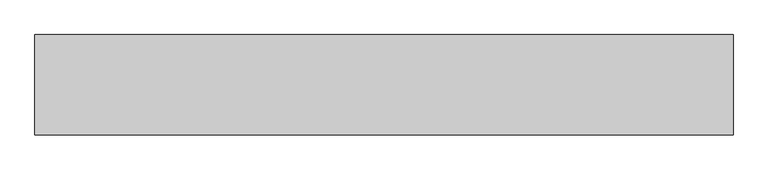
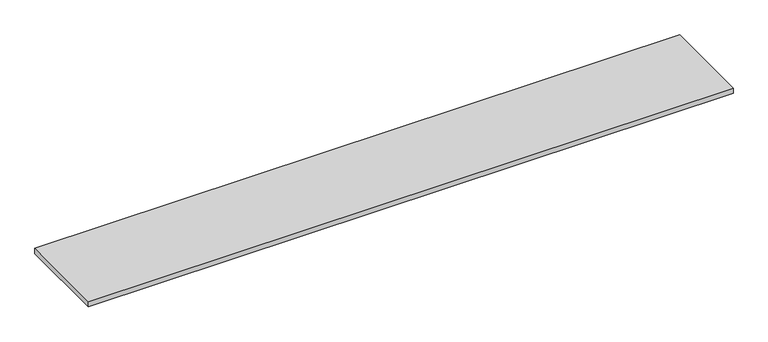
"""IFC4 building model written with IfcOpenShell, lengths in millimetres: furniture geometry, OD_CW_Countertop : OD_CW_Countertop."""

from ifc_helpers import new_model, si_unit, frame, origin, place, context, project, spatial, polyline, outline, extrude, source, transform, mapped, element, save


def furniture_1b7fe929(model_context):
    return source(origin(), model_context, "Body", "SweptSolid", [
        extrude(outline(polyline([(18.7377049, -609.6), (18.7377049, 25.4), (4438.3377049, 25.4), (4438.3377049, -609.6), (18.7377049, -609.6)])), frame((0.0, 0.0, 965.2), z_axis=(0.0, 0.0, 1.0), x_axis=(1.0, 0.0, 0.0)), (0.0, 0.0, 1.0), 38.1),
    ])


if __name__ == "__main__":
    model = new_model("IFC4")
    model_context = context("Model", 3, world=origin())
    ifc_project = project(units=[si_unit("LENGTHUNIT", "METRE", prefix="MILLI")], contexts=[model_context])
    site = spatial("IfcSite", under=ifc_project)
    building = spatial("IfcBuilding", under=site)
    placement = place(None, origin())
    furniture_shape = furniture_1b7fe929(model_context)
    element("IfcFurniture", 1, ObjectType="OD_CW_Countertop : OD_CW_Countertop", at=placement, inside=building, context=model_context, shape_type="MappedRepresentation", body=[
        mapped(furniture_shape, transform((0.0, 0.0, 0.0), x_axis=(1.0, 0.0, 0.0), y_axis=(0.0, 1.0, 0.0), z_axis=(0.0, 0.0, 1.0))),
    ])
    save(model, "model.ifc")

# Revit data of these elements
# Type "OD_CW_Countertop : OD_CW_Countertop"
#   OD_CW_Width [instance default] = 2' - 9"
#   OD_CW_Off Floor [instance default] = 3' - 2"
#   OD_CW_Length [instance default] = 6' - 9"
#   OD_CW_Height [instance default] = 7' - 0"
#   Depth = 2' - 0"
#   Height = 3' - 0"
#   Width = 4' - 0"
#   OD_CW_Material_Countertop [instance default] = none
# Element 1 (IfcFurniture, "OD_CW_Countertop : OD_CW_Countertop")
#   OD_CW_Width = 2' - 1"
#   OD_CW_Length = 14' - 6"
#   OD_CW_Height = 0' - 1 1/2"
#   Materials on its faces: "CASEWORK"
# Materials
#   "CASEWORK": class "Generic", colour RGB 181 181 181, transparency 0, Cost = 0
